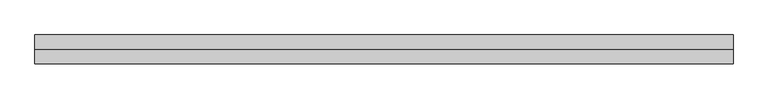
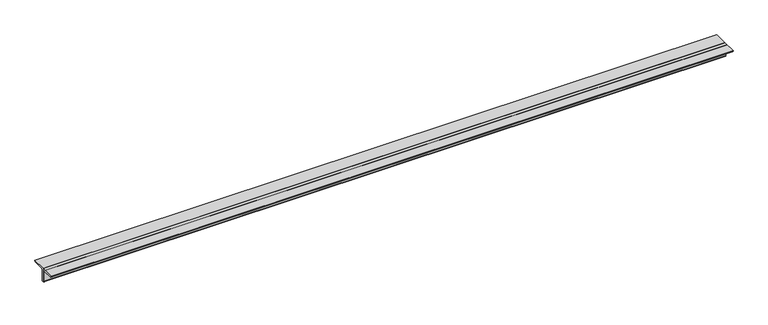
"""IFC4 building model written with IfcOpenShell, lengths in millimetres: beam geometry, 0123_Steel Framing_2Ls-KSD3502 : H_SB_AR_S04_2Ls-130x130x12_VBR2."""

from ifc_helpers import new_model, si_unit, point, frame, frame_2d, origin, place, context, project, spatial, polyline, circle_curve, trimmed, segment, composite_curve, outline, extrude, source, transform, mapped, element, save


def beam_08074ba6(model_context):
    return source(origin(), model_context, "Body", "SweptSolid", [
        extrude(outline(composite_curve([segment(polyline([(0.0, 36.4), (130.0, 36.4)]), True, "CONTINUOUS"), segment(trimmed(circle_curve(frame_2d((118.0, 36.4)), 12.0), [point((130.0, 36.4))], [point((118.0, 24.4))], False, "CARTESIAN"), True, "CONTINUOUS"), segment(polyline([(118.0, 24.4), (24.0, 24.4)]), True, "CONTINUOUS"), segment(trimmed(circle_curve(frame_2d((24.0, 12.4)), 12.0), [point((24.0, 24.4))], [point((12.0, 12.4))], True, "CARTESIAN"), True, "CONTINUOUS"), segment(polyline([(12.0, 12.4), (12.0, -81.6)]), True, "CONTINUOUS"), segment(trimmed(circle_curve(frame_2d((0.0, -81.6)), 12.0), [point((12.0, -81.6))], [point((0.0, -93.6))], False, "CARTESIAN"), True, "CONTINUOUS"), segment(polyline([(0.0, -93.6), (0.0, 36.4)]), True, "CONTINUOUS")], self_intersect=False)), frame((-2961.9806044, 0.0, 0.0), z_axis=(1.0, 0.0, 0.0), x_axis=(0.0, 1.0, 0.0)), (0.0, 0.0, 1.0), 6322.5847795),
        extrude(outline(composite_curve([segment(polyline([(0.0, 36.4), (0.0, -93.6)]), True, "CONTINUOUS"), segment(trimmed(circle_curve(frame_2d((0.0, -81.6)), 12.0), [point((0.0, -93.6))], [point((-12.0, -81.6))], False, "CARTESIAN"), True, "CONTINUOUS"), segment(polyline([(-12.0, -81.6), (-12.0, 12.4)]), True, "CONTINUOUS"), segment(trimmed(circle_curve(frame_2d((-24.0, 12.4)), 12.0), [point((-12.0, 12.4))], [point((-24.0, 24.4))], True, "CARTESIAN"), True, "CONTINUOUS"), segment(polyline([(-24.0, 24.4), (-118.0, 24.4)]), True, "CONTINUOUS"), segment(trimmed(circle_curve(frame_2d((-118.0, 36.4)), 12.0), [point((-118.0, 24.4))], [point((-130.0, 36.4))], False, "CARTESIAN"), True, "CONTINUOUS"), segment(polyline([(-130.0, 36.4), (0.0, 36.4)]), True, "CONTINUOUS")], self_intersect=False)), frame((-2961.9806044, 0.0, 0.0), z_axis=(1.0, 0.0, 0.0), x_axis=(0.0, 1.0, 0.0)), (0.0, 0.0, 1.0), 6322.5847795),
    ])


if __name__ == "__main__":
    model = new_model("IFC4")
    model_context = context("Model", 3, world=origin())
    ifc_project = project(units=[si_unit("LENGTHUNIT", "METRE", prefix="MILLI")], contexts=[model_context])
    site = spatial("IfcSite", under=ifc_project)
    building = spatial("IfcBuilding", under=site)
    placement = place(None, origin())
    beam_shape = beam_08074ba6(model_context)
    element("IfcBeam", 1, ObjectType="0123_Steel Framing_2Ls-KSD3502 : H_SB_AR_S04_2Ls-130x130x12_VBR2", at=placement, inside=building, context=model_context, shape_type="MappedRepresentation", body=[
        mapped(beam_shape, transform((0.0, 0.0, 0.0), x_axis=(1.0, 0.0, 0.0), y_axis=(0.0, 1.0, 0.0), z_axis=(0.0, 0.0, 1.0))),
    ])
    save(model, "model.ifc")

# Revit data of these elements
# Type "0123_Steel Framing_2Ls-KSD3502 : H_SB_AR_S04_2Ls-130x130x12_VBR2"
#   Type Mark = "VBR2"
#   Assembly Code = "B10"
#   Legs = "SLBB"
#   W = 8.97
#   Perimeter = 1.04 m²/m
#   Nominal Weight = 46.80 kgf/m
#   Length [instance default] = 1000 mm
#   Space = 0 mm
#   b = 130 mm
#   d = 130 mm
#   t = 12 mm
#   y = 36.4 mm
#   A = 0.005952 m²
#   Structural Material [instance default] = Steel ASTM A36
# Element 1 (IfcBeam, "0123_Steel Framing_2Ls-KSD3502 : H_SB_AR_S04_2Ls-130x130x12_VBR2")
#   Materials on its faces: "Steel ASTM A36"
# Materials
#   "Steel ASTM A36": class "Metal", colour RGB 199 199 199, transparency 0, Description = "Structural steel, ASTM A36 Grade B, mill finish", Cost = 0
